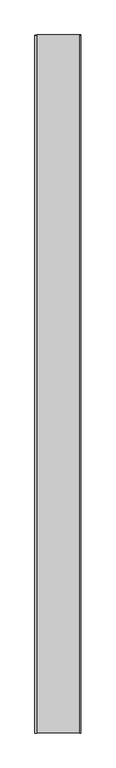
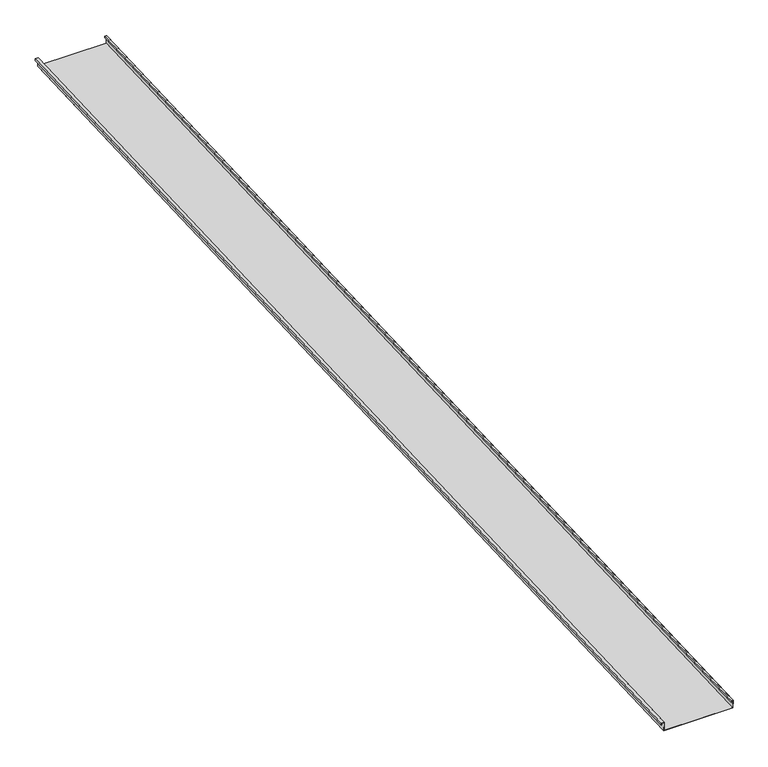
"""IFC4 building model written with IfcOpenShell, lengths in millimetres: proxy geometry, Generic Models 2:Generic Models 2:310765:Generic Models 2:310765 : Generic Models 2:Generic Models 2:310765:119 : Generic Models 2:Generic Models 2:310765:Generic Models 2:310765 : Generic Models 2:Generic Models 2:310765:300385."""

from ifc_helpers import new_model, si_unit, frame, origin, place, context, project, spatial, polyline, outline, extrude, source, transform, mapped, element, save


def generic_models_a7abbb59(model_context):
    return source(origin(), model_context, "Body", "SweptSolid", [
        extrude(outline(polyline([(1.5875, 0.0), (1.5875, 50.8), (407.9875, 50.8), (407.9875, 1.5875), (396.875, 1.5875), (396.875, 11.1125), (398.4625, 11.1125), (398.4625, 3.175), (406.4, 3.175), (406.4, 49.2125), (3.175, 49.2125), (3.175, -1.5874999), (-14.2875, -1.5874999), (-14.2875, 9.525), (-12.7, 9.525), (-12.7, 0.0), (1.5875, 0.0)])), frame((665843.6596405, -581354.4345603, 3902.6697972), z_axis=(0.0, 0.9991330730923568, 0.041630544712067834), x_axis=(1.0, 0.0, 0.0)), (0.0, 0.0, 1.0), 6400.8),
    ])


if __name__ == "__main__":
    model = new_model("IFC4")
    model_context = context("Model", 3, world=origin())
    ifc_project = project(units=[si_unit("LENGTHUNIT", "METRE", prefix="MILLI")], contexts=[model_context])
    site = spatial("IfcSite", under=ifc_project)
    building = spatial("IfcBuilding", under=site)
    placement = place(None, origin())
    generic_models_shape = generic_models_a7abbb59(model_context)
    element("IfcBuildingElementProxy", 1, Name="Generic Models 2:Generic Models 2:310765:Generic Models 2:310765 : Generic Models 2:Generic Models 2:310765:119 : Generic Models 2:Generic Models 2:310765:Generic Models 2:310765 : Generic Models 2:Generic Models 2:310765:300385", ObjectType="Generic Models 2:Generic Models 2:310765:Generic Models 2:310765 : Generic Models 2:Generic Models 2:310765:119 : Generic Models 2:Generic Models 2:310765:Generic Models 2:310765 : Generic Models 2:Generic Models 2:310765:300385", at=placement, inside=building, context=model_context, shape_type="MappedRepresentation", body=[
        mapped(generic_models_shape, transform((0.0, 0.0, 0.0), x_axis=(1.0, 0.0, 0.0), y_axis=(0.0, 1.0, 0.0), z_axis=(0.0, 0.0, 1.0))),
    ])
    save(model, "model.ifc")

# Revit data of these elements
# Type "Generic Models 2:Generic Models 2:310765:Generic Models 2:310765 : Generic Models 2:Generic Models 2:310765:119 : Generic Models 2:Generic Models 2:310765:Generic Models 2:310765 : Generic Models 2:Generic Models 2:310765:300385"
#   NameOverride = "Generic Models 2:Generic Models 2:310765:Generic Models 2:310765 : Generic Models 2:Generic Models 2:310765:300385"
#   ObjectTypeOverride = "Generic Models 2:310765 : Generic Models 2:Generic Models 2:310765"
#   Reference = "Generic Models 2"
#   Tag = "300385"
# Element 1 (IfcBuildingElementProxy, "Generic Models 2:Generic Models 2:310765:Generic Models 2:310765 : Generic Models 2:Generic Models 2:310765:119 : Generic Models 2:Generic Models 2:310765:Generic Models 2:310765 : Generic Models 2:Generic Models 2:310765:300385")
#   Materials on its faces: "THERMAL BROKEN ALUMINUM STOREFRONT FOR POLYCARBONATE"
# Materials
#   "THERMAL BROKEN ALUMINUM STOREFRONT FOR POLYCARBONATE": class "Unassigned", colour RGB 244 244 244, transparency 0, Keynote = "M07611300.01", Cost = 0
